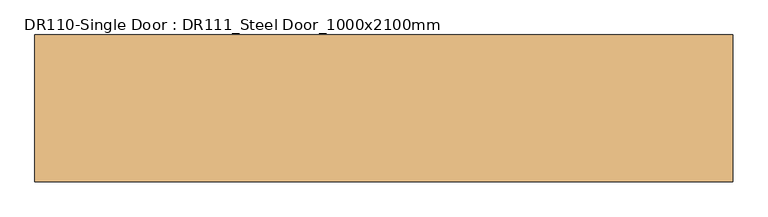
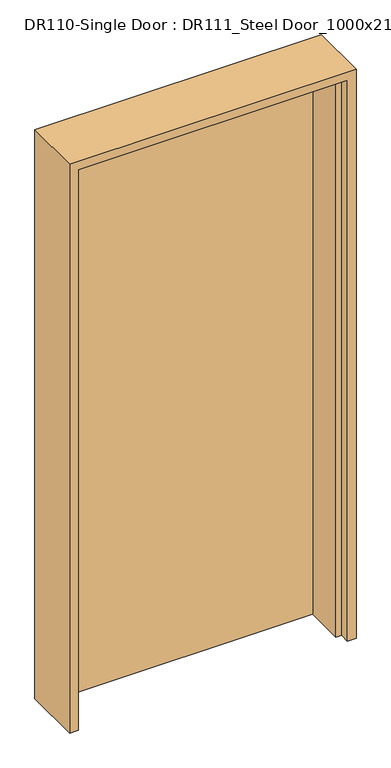
"""IFC4 building model written with IfcOpenShell, lengths in millimetres: door geometry, DR110-Single Door : DR111_Steel Door_1000x2100mm."""

from ifc_helpers import new_model, si_unit, origin, origin_with_axes, place, context, project, spatial, polyline, outline, extrude, faceted_brep, source, transform, mapped, element, save


def dr110_single_door_dr111_steel_door_1000x2100mm_6218e75e(model_context):
    return source(origin(), model_context, "Body", "SolidModel", [
        extrude(outline(polyline([(470.0, 105.0), (470.0, 70.0), (-470.0, 70.0), (-470.0, 105.0), (470.0, 105.0)])), origin_with_axes(), (0.0, 0.0, 1.0), 2070.0),
        faceted_brep([(470.0, 105.0, 0.0), (500.0, 105.0, 0.0), (500.0, -105.0, 0.0), (470.0, -105.0, 0.0), (470.0, -70.0, 0.0), (450.0, -70.0, 0.0), (450.0, 70.0, 0.0), (470.0, 70.0, 0.0), (470.0, 105.0, 2070.0), (-470.0, 105.0, 2070.0), (-470.0, 105.0, 0.0), (-500.0, 105.0, 0.0), (-500.0, 105.0, 2100.0), (500.0, 105.0, 2100.0), (500.0, -105.0, 2100.0), (-500.0, -105.0, 2100.0), (-500.0, -105.0, 0.0), (-470.0, -105.0, 0.0), (-470.0, -105.0, 2070.0), (470.0, -105.0, 2070.0), (470.0, -70.0, 2070.0), (-470.0, -70.0, 2070.0), (-470.0, -70.0, 0.0), (-450.0, -70.0, 0.0), (-450.0, -70.0, 2050.0), (450.0, -70.0, 2050.0), (450.0, 70.0, 2050.0), (-450.0, 70.0, 2050.0), (-450.0, 70.0, 0.0), (-470.0, 70.0, 0.0), (-470.0, 70.0, 2070.0), (470.0, 70.0, 2070.0)], [[[0, 1, 2, 3, 4, 5, 6, 7]], [[1, 0, 8, 9, 10, 11, 12, 13]], [[2, 1, 13, 14]], [[3, 2, 14, 15, 16, 17, 18, 19]], [[4, 3, 19, 20]], [[5, 4, 20, 21, 22, 23, 24, 25]], [[6, 5, 25, 26]], [[7, 6, 26, 27, 28, 29, 30, 31]], [[0, 7, 31, 8]], [[9, 30, 29, 10]], [[10, 29, 28, 23, 22, 17, 16, 11]], [[15, 12, 11, 16]], [[21, 18, 17, 22]], [[27, 24, 23, 28]], [[14, 13, 12, 15]], [[20, 19, 18, 21]], [[26, 25, 24, 27]], [[8, 31, 30, 9]]]),
    ])


if __name__ == "__main__":
    model = new_model("IFC4")
    model_context = context("Model", 3, world=origin())
    ifc_project = project(units=[si_unit("LENGTHUNIT", "METRE", prefix="MILLI")], contexts=[model_context])
    site = spatial("IfcSite", under=ifc_project)
    building = spatial("IfcBuilding", under=site)
    placement = place(None, origin())
    dr110_single_door_dr111_steel_door_1000x2100mm_shape = dr110_single_door_dr111_steel_door_1000x2100mm_6218e75e(model_context)
    element("IfcDoor", 1, ObjectType="DR110-Single Door : DR111_Steel Door_1000x2100mm", at=placement, inside=building, context=model_context, shape_type="MappedRepresentation", body=[
        mapped(dr110_single_door_dr111_steel_door_1000x2100mm_shape, transform((0.0, 0.0, 0.0), x_axis=(1.0, 0.0, 0.0), y_axis=(0.0, 1.0, 0.0), z_axis=(0.0, 0.0, 1.0))),
    ])
    save(model, "model.ifc")

# Revit data of these elements
# Type "DR110-Single Door : DR111_Steel Door_1000x2100mm"
#   Type Mark = "SD"
#   Analytic Construction = "<None>"
#   프레임 투영 외부. = 25 mm
#   프레임 투영 내부. = 25 mm
#   프레임 폭 = 75 mm
#   Height = 2100 mm
#   Width = 1000 mm
#   Define Thermal Properties by = 1
#   문 패널 = none
#   문 프레임 = A04AQ098-00002_Steel Door_non FP_single
#   Function = (empty or 0)
#   Wall Closure = (empty or 0)
# Element 1 (IfcDoor, "DR110-Single Door : DR111_Steel Door_1000x2100mm")
#   Materials on its faces: "A04AQ098-00002_Steel Door_non FP_single"
# Materials
#   "A04AQ098-00002_Steel Door_non FP_single": class "금속", colour RGB 247 247 247, transparency 0, Description = "Steel Door", W00) Work Master Code = "A04AQ098-00002", W01) Work Master_Lv1 = "Finishing Work", W02) Work Master_Lv2 = "Door & Window Work", W03) Work Master_Spec.1 = "Steel Door w/ Steel Frame", W04) Work Master_Spec.2 = "Fire Protective Rating: N/A, Single Door", W05) Work Master_Spec.3 = "w/ Hardware & Accessories", Cost = 0
